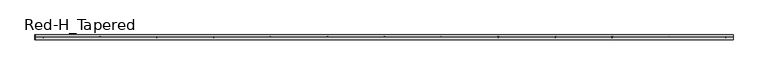
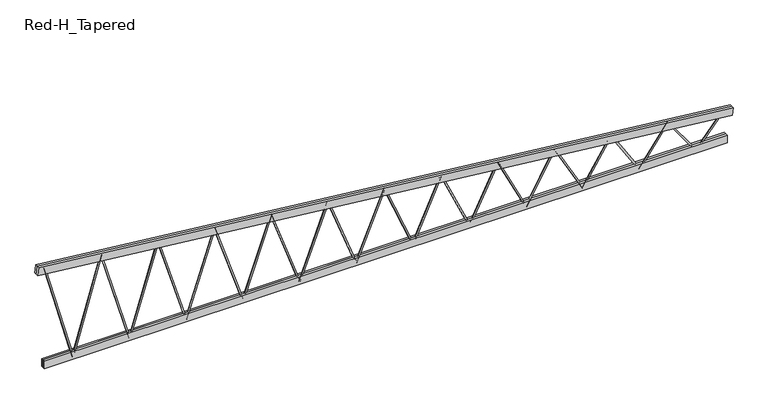
"""IFC4 building model written with IfcOpenShell, lengths in millimetres: beam geometry, Construction_Frames_RedBuilt_Openweb_Red-H_Tapered : Red-H_Tapered."""

from ifc_helpers import new_model, si_unit, point, frame, origin, origin_2d, place, context, project, spatial, polyline, circle_curve, trimmed, segment, composite_curve, outline, extrude, source, transform, mapped, element, save


def red_h_tapered_b2b48a9a(model_context):
    return source(origin(), model_context, "Body", "SweptSolid", [
        extrude(outline(composite_curve([segment(trimmed(circle_curve(origin_2d(), 12.7), [point((0.0, -12.7))], [point((0.0, 12.7))], False, "CARTESIAN"), True, "CONTINUOUS"), segment(trimmed(circle_curve(origin_2d(), 12.7), [point((0.0, 12.7))], [point((0.0, -12.7))], False, "CARTESIAN"), True, "CONTINUOUS")], self_intersect=False)), frame((-491.6619792, 0.0, -367.0101562), z_axis=(-0.35578994847905354, 0.0, 0.9345659487490824), x_axis=(0.0, -1.0, 0.0)), (0.0, 0.0, 1.0), 1381.888334),
        extrude(outline(composite_curve([segment(trimmed(circle_curve(origin_2d(), 12.7), [point((0.0, 12.7))], [point((0.0, -12.6999999))], False, "CARTESIAN"), True, "CONTINUOUS"), segment(trimmed(circle_curve(origin_2d(), 12.7), [point((0.0, -12.6999999))], [point((0.0, 12.7))], False, "CARTESIAN"), True, "CONTINUOUS")], self_intersect=False)), frame((-1474.9859375, 0.0, -367.0101562), z_axis=(0.3557899484790537, 0.0, 0.9345659487490823), x_axis=(0.0, -1.0, 0.0)), (0.0, 0.0, 1.0), 1381.888334),
        extrude(outline(composite_curve([segment(trimmed(circle_curve(origin_2d(), 12.7), [point((0.0, -12.7))], [point((0.0, 12.6999999))], False, "CARTESIAN"), True, "CONTINUOUS"), segment(trimmed(circle_curve(origin_2d(), 12.7), [point((0.0, 12.6999999))], [point((0.0, -12.7))], False, "CARTESIAN"), True, "CONTINUOUS")], self_intersect=False)), frame((-1474.9859375, 0.0, -367.0101562), z_axis=(-0.3329345647396236, 0.0, 0.9429499327120382), x_axis=(0.0, -1.0, 0.0)), (0.0, 0.0, 1.0), 1476.7525852),
        extrude(outline(composite_curve([segment(trimmed(circle_curve(origin_2d(), 12.7), [point((0.0, -12.7))], [point((0.0, 12.7))], False, "CARTESIAN"), True, "CONTINUOUS"), segment(trimmed(circle_curve(origin_2d(), 12.7), [point((0.0, 12.7))], [point((0.0, -12.7))], False, "CARTESIAN"), True, "CONTINUOUS")], self_intersect=False)), frame((-2458.3098958, 0.0, -367.0101562), z_axis=(0.3329345647396277, 0.0, 0.9429499327120368), x_axis=(0.0, -1.0, 0.0)), (0.0, 0.0, 1.0), 1476.7525852),
        extrude(outline(composite_curve([segment(trimmed(circle_curve(origin_2d(), 12.7), [point((0.0, 12.7))], [point((0.0, -12.7))], False, "CARTESIAN"), True, "CONTINUOUS"), segment(trimmed(circle_curve(origin_2d(), 12.7), [point((0.0, -12.7))], [point((0.0, 12.7))], False, "CARTESIAN"), True, "CONTINUOUS")], self_intersect=False)), frame((-2458.3098958, 0.0, -367.0101562), z_axis=(-0.31268525401434294, 0.0, 0.9498567954812904), x_axis=(0.0, -1.0, 0.0)), (0.0, 0.0, 1.0), 1572.3862026),
        extrude(outline(composite_curve([segment(trimmed(circle_curve(origin_2d(), 12.7), [point((0.0, -12.7))], [point((0.0, 12.7))], False, "CARTESIAN"), True, "CONTINUOUS"), segment(trimmed(circle_curve(origin_2d(), 12.7), [point((0.0, 12.7))], [point((0.0, -12.7))], False, "CARTESIAN"), True, "CONTINUOUS")], self_intersect=False)), frame((-3441.6338542, 0.0, -367.0101562), z_axis=(0.31268525401434244, 0.0, 0.9498567954812905), x_axis=(0.0, -1.0, 0.0)), (0.0, 0.0, 1.0), 1572.3862026),
        extrude(outline(composite_curve([segment(trimmed(circle_curve(origin_2d(), 12.7), [point((0.0, 12.7))], [point((0.0, -12.7))], False, "CARTESIAN"), True, "CONTINUOUS"), segment(trimmed(circle_curve(origin_2d(), 12.7), [point((0.0, -12.7))], [point((0.0, 12.7))], False, "CARTESIAN"), True, "CONTINUOUS")], self_intersect=False)), frame((-3441.6338542, 0.0, -367.0101562), z_axis=(-0.2946453378709869, 0.0, 0.9556066789589177), x_axis=(0.0, -1.0, 0.0)), (0.0, 0.0, 1.0), 1668.6569104),
        extrude(outline(composite_curve([segment(trimmed(circle_curve(origin_2d(), 12.7), [point((0.0, -12.7))], [point((0.0, 12.7))], False, "CARTESIAN"), True, "CONTINUOUS"), segment(trimmed(circle_curve(origin_2d(), 12.7), [point((0.0, 12.7))], [point((0.0, -12.7))], False, "CARTESIAN"), True, "CONTINUOUS")], self_intersect=False)), frame((-4424.9578125, 0.0, -367.0101562), z_axis=(0.29464533787099256, 0.0, 0.9556066789589159), x_axis=(0.0, -1.0, 0.0)), (0.0, 0.0, 1.0), 1668.6569104),
        extrude(outline(composite_curve([segment(trimmed(circle_curve(origin_2d(), 12.7), [point((0.0, 12.7))], [point((0.0, -12.7))], False, "CARTESIAN"), True, "CONTINUOUS"), segment(trimmed(circle_curve(origin_2d(), 12.7), [point((0.0, -12.7))], [point((0.0, 12.7))], False, "CARTESIAN"), True, "CONTINUOUS")], self_intersect=False)), frame((-4424.9578125, 0.0, -367.0101562), z_axis=(-0.2784893697457482, 0.0, 0.9604393114292105), x_axis=(0.0, -1.0, 0.0)), (0.0, 0.0, 1.0), 1765.46049),
        extrude(outline(composite_curve([segment(trimmed(circle_curve(origin_2d(), 12.7), [point((0.0, -12.7))], [point((0.0, 12.6999999))], False, "CARTESIAN"), True, "CONTINUOUS"), segment(trimmed(circle_curve(origin_2d(), 12.7), [point((0.0, 12.6999999))], [point((0.0, -12.7))], False, "CARTESIAN"), True, "CONTINUOUS")], self_intersect=False)), frame((-5408.2817708, 0.0, -367.0101562), z_axis=(0.27848936974574684, 0.0, 0.9604393114292109), x_axis=(0.0, -1.0, 0.0)), (0.0, 0.0, 1.0), 1765.46049),
        extrude(outline(composite_curve([segment(trimmed(circle_curve(origin_2d(), 12.7), [point((0.0, 12.7))], [point((0.0, -12.7000001))], False, "CARTESIAN"), True, "CONTINUOUS"), segment(trimmed(circle_curve(origin_2d(), 12.7), [point((0.0, -12.7000001))], [point((0.0, 12.7))], False, "CARTESIAN"), True, "CONTINUOUS")], self_intersect=False)), frame((-5408.2817708, 0.0, -367.0101562), z_axis=(-0.2639492777400827, 0.0, 0.9645365616608262), x_axis=(0.0, -1.0, 0.0)), (0.0, 0.0, 1.0), 1862.7138645),
        extrude(outline(composite_curve([segment(trimmed(circle_curve(origin_2d(), 12.7), [point((0.0, 12.7000001))], [point((0.0, -12.6999999))], False, "CARTESIAN"), True, "CONTINUOUS"), segment(trimmed(circle_curve(origin_2d(), 12.7), [point((0.0, -12.6999999))], [point((0.0, 12.7000001))], False, "CARTESIAN"), True, "CONTINUOUS")], self_intersect=False)), frame((5408.2817708, 0.0, -367.0101562), z_axis=(0.6439089672678159, 0.0, 0.7651021120557013), x_axis=(0.0, -1.0, 0.0)), (0.0, 0.0, 1.0), 763.5582111),
        extrude(outline(composite_curve([segment(trimmed(circle_curve(origin_2d(), 12.7), [point((0.0, -12.7))], [point((0.0, 12.7))], False, "CARTESIAN"), True, "CONTINUOUS"), segment(trimmed(circle_curve(origin_2d(), 12.7), [point((0.0, 12.7))], [point((0.0, -12.7))], False, "CARTESIAN"), True, "CONTINUOUS")], self_intersect=False)), frame((5408.2817708, 0.0, -367.0101562), z_axis=(-0.582969105772275, 0.0, 0.8124943210355837), x_axis=(0.0, -1.0, 0.0)), (0.0, 0.0, 1.0), 843.3757026),
        extrude(outline(composite_curve([segment(trimmed(circle_curve(origin_2d(), 12.7), [point((0.0, 12.7000001))], [point((0.0, -12.7))], False, "CARTESIAN"), True, "CONTINUOUS"), segment(trimmed(circle_curve(origin_2d(), 12.7), [point((0.0, -12.7))], [point((0.0, 12.7000001))], False, "CARTESIAN"), True, "CONTINUOUS")], self_intersect=False)), frame((4424.9578125, 0.0, -367.0101562), z_axis=(0.5829691057722728, 0.0, 0.8124943210355852), x_axis=(0.0, -1.0, 0.0)), (0.0, 0.0, 1.0), 843.3757026),
        extrude(outline(composite_curve([segment(trimmed(circle_curve(origin_2d(), 12.7), [point((0.0, -12.7))], [point((0.0, 12.6999999))], False, "CARTESIAN"), True, "CONTINUOUS"), segment(trimmed(circle_curve(origin_2d(), 12.7), [point((0.0, 12.6999999))], [point((0.0, -12.7))], False, "CARTESIAN"), True, "CONTINUOUS")], self_intersect=False)), frame((4424.9578125, 0.0, -367.0101562), z_axis=(-0.530184660192729, 0.0, 0.8478822006011923), x_axis=(0.0, -1.0, 0.0)), (0.0, 0.0, 1.0), 927.3410117),
        extrude(outline(composite_curve([segment(trimmed(circle_curve(origin_2d(), 12.7), [point((0.0, 12.7))], [point((0.0, -12.7))], False, "CARTESIAN"), True, "CONTINUOUS"), segment(trimmed(circle_curve(origin_2d(), 12.7), [point((0.0, -12.7))], [point((0.0, 12.7))], False, "CARTESIAN"), True, "CONTINUOUS")], self_intersect=False)), frame((3441.6338542, 0.0, -367.0101562), z_axis=(0.5301846601927269, 0.0, 0.8478822006011937), x_axis=(0.0, -1.0, 0.0)), (0.0, 0.0, 1.0), 927.3410117),
        extrude(outline(composite_curve([segment(trimmed(circle_curve(origin_2d(), 12.7), [point((0.0, -12.7))], [point((0.0, 12.7))], False, "CARTESIAN"), True, "CONTINUOUS"), segment(trimmed(circle_curve(origin_2d(), 12.7), [point((0.0, 12.7))], [point((0.0, -12.7))], False, "CARTESIAN"), True, "CONTINUOUS")], self_intersect=False)), frame((3441.6338542, 0.0, -367.0101562), z_axis=(-0.48467074935534127, 0.0, 0.8746966701201806), x_axis=(0.0, -1.0, 0.0)), (0.0, 0.0, 1.0), 1014.4246993),
        extrude(outline(composite_curve([segment(trimmed(circle_curve(origin_2d(), 12.7), [point((0.0, 12.7))], [point((0.0, -12.7))], False, "CARTESIAN"), True, "CONTINUOUS"), segment(trimmed(circle_curve(origin_2d(), 12.7), [point((0.0, -12.7))], [point((0.0, 12.7))], False, "CARTESIAN"), True, "CONTINUOUS")], self_intersect=False)), frame((2458.3098958, 0.0, -367.0101562), z_axis=(0.48467074935534193, 0.0, 0.8746966701201804), x_axis=(0.0, -1.0, 0.0)), (0.0, 0.0, 1.0), 1014.4246993),
        extrude(outline(composite_curve([segment(trimmed(circle_curve(origin_2d(), 12.7), [point((0.0, -12.7))], [point((0.0, 12.7))], False, "CARTESIAN"), True, "CONTINUOUS"), segment(trimmed(circle_curve(origin_2d(), 12.7), [point((0.0, 12.7))], [point((0.0, -12.7))], False, "CARTESIAN"), True, "CONTINUOUS")], self_intersect=False)), frame((2458.3098958, 0.0, -367.0101562), z_axis=(-0.4453907754718369, 0.0, 0.8953362815861959), x_axis=(0.0, -1.0, 0.0)), (0.0, 0.0, 1.0), 1103.8890032),
        extrude(outline(composite_curve([segment(trimmed(circle_curve(origin_2d(), 12.7), [point((0.0, 12.7))], [point((0.0, -12.7))], False, "CARTESIAN"), True, "CONTINUOUS"), segment(trimmed(circle_curve(origin_2d(), 12.7), [point((0.0, -12.7))], [point((0.0, 12.7))], False, "CARTESIAN"), True, "CONTINUOUS")], self_intersect=False)), frame((1474.9859375, 0.0, -367.0101562), z_axis=(0.445390775471841, 0.0, 0.8953362815861938), x_axis=(0.0, -1.0, 0.0)), (0.0, 0.0, 1.0), 1103.8890032),
        extrude(outline(composite_curve([segment(trimmed(circle_curve(origin_2d(), 12.7), [point((0.0, -12.7))], [point((0.0, 12.7))], False, "CARTESIAN"), True, "CONTINUOUS"), segment(trimmed(circle_curve(origin_2d(), 12.7), [point((0.0, 12.7))], [point((0.0, -12.7))], False, "CARTESIAN"), True, "CONTINUOUS")], self_intersect=False)), frame((1474.9859375, 0.0, -367.0101562), z_axis=(-0.41136395902525497, 0.0, 0.9114711697114004), x_axis=(0.0, -1.0, 0.0)), (0.0, 0.0, 1.0), 1195.1994539),
        extrude(outline(composite_curve([segment(trimmed(circle_curve(origin_2d(), 12.7), [point((0.0, 12.7))], [point((0.0, -12.7))], False, "CARTESIAN"), True, "CONTINUOUS"), segment(trimmed(circle_curve(origin_2d(), 12.7), [point((0.0, -12.7))], [point((0.0, 12.7))], False, "CARTESIAN"), True, "CONTINUOUS")], self_intersect=False)), frame((491.6619792, 0.0, -367.0101562), z_axis=(0.41136395902525574, 0.0, 0.9114711697114), x_axis=(0.0, -1.0, 0.0)), (0.0, 0.0, 1.0), 1195.1994539),
        extrude(outline(composite_curve([segment(trimmed(circle_curve(origin_2d(), 12.7), [point((0.0, -12.7))], [point((0.0, 12.7))], False, "CARTESIAN"), True, "CONTINUOUS"), segment(trimmed(circle_curve(origin_2d(), 12.7), [point((0.0, 12.7))], [point((0.0, -12.7))], False, "CARTESIAN"), True, "CONTINUOUS")], self_intersect=False)), frame((491.6619792, 0.0, -367.0101562), z_axis=(-0.3817359681353622, 0.0, 0.9242714161066314), x_axis=(0.0, -1.0, 0.0)), (0.0, 0.0, 1.0), 1287.9634622),
        extrude(outline(composite_curve([segment(trimmed(circle_curve(origin_2d(), 12.7), [point((0.0, 12.7))], [point((0.0, -12.7))], False, "CARTESIAN"), True, "CONTINUOUS"), segment(trimmed(circle_curve(origin_2d(), 12.7), [point((0.0, -12.7))], [point((0.0, 12.7))], False, "CARTESIAN"), True, "CONTINUOUS")], self_intersect=False)), frame((-491.6619792, 0.0, -367.0101562), z_axis=(0.3817359681353307, 0.0, 0.9242714161066444), x_axis=(0.0, -1.0, 0.0)), (0.0, 0.0, 1.0), 1287.9634622),
        extrude(outline(polyline([(-5925.34375, -41.275), (-5925.34375, -3.175), (5925.34375, -3.175), (5925.34375, -41.275), (-5925.34375, -41.275)])), frame((0.0, 0.0, -386.0601562), z_axis=(0.0, 0.0, 1.0), x_axis=(1.0, 0.0, 0.0)), (0.0, 0.0, 1.0), 139.7),
        extrude(outline(polyline([(-5925.34375, 3.175), (-5925.34375, 41.275), (5925.34375, 41.275), (5925.34375, 3.175), (-5925.34375, 3.175)])), frame((0.0, 0.0, -386.0601562), z_axis=(0.0, 0.0, 1.0), x_axis=(1.0, 0.0, 0.0)), (0.0, 0.0, 1.0), 139.7),
        extrude(outline(polyline([(0.0, -38.1), (0.0, 0.0), (12121.9438686, 0.0), (12121.9438686, -38.1), (0.0, -38.1)])), frame((-6041.7262958, -3.175, 1367.3241631), z_axis=(0.10581636195546858, 0.0, 0.9943856885245832), x_axis=(0.9943856885245832, 0.0, -0.10581636195546858)), (0.0, 0.0, 1.0), 139.7),
        extrude(outline(polyline([(0.0, -38.1), (0.0, 0.0), (12121.9438686, 0.0), (12121.9438686, -38.1), (0.0, -38.1)])), frame((-6041.7262958, 41.275, 1367.3241631), z_axis=(0.10581636195546858, 0.0, 0.9943856885245832), x_axis=(0.9943856885245832, 0.0, -0.10581636195546858)), (0.0, 0.0, 1.0), 139.7),
    ])


if __name__ == "__main__":
    model = new_model("IFC4")
    model_context = context("Model", 3, world=origin())
    ifc_project = project(units=[si_unit("LENGTHUNIT", "METRE", prefix="MILLI")], contexts=[model_context])
    site = spatial("IfcSite", under=ifc_project)
    building = spatial("IfcBuilding", under=site)
    placement = place(None, origin())
    red_h_tapered_shape = red_h_tapered_b2b48a9a(model_context)
    element("IfcBeam", 1, ObjectType="Construction_Frames_RedBuilt_Openweb_Red-H_Tapered : Red-H_Tapered", at=placement, inside=building, context=model_context, shape_type="MappedRepresentation", body=[
        mapped(red_h_tapered_shape, transform((0.0, 0.0, 0.0), x_axis=(1.0, 0.0, 0.0), y_axis=(0.0, 1.0, 0.0), z_axis=(0.0, 0.0, 1.0))),
    ])
    save(model, "model.ifc")

# Revit data of these elements
# Type "Construction_Frames_RedBuilt_Openweb_Red-H_Tapered : Red-H_Tapered"
#   Youtube clip = ""
#   Weight Net (Kg) = "0"
#   Webs = "Up to 2\" diameter tubular steel"
#   Uniformat II Description = ""
#   Uniformat II Code = ""
#   Uniclass 2015 Name = "Softwood trusses"
#   Uniclass 2015 Code = "Pr_20_85_90_81"
#   Uniclass 2.0 Description = "Structural Framing Systems"
#   Uniclass 2.0 Code = "SS-15-10-75"
#   Uniclass 1.4 Description = "Trusses"
#   Uniclass 1.4 Code = "L3523"
#   UNSPSC Code = "30103606"
#   Technical description = "http://www.redbuilt.com/reference/literature-and-other-resources"
#   Region South America = "None"
#   Region Oceania = "None"
#   Region North America = "US"
#   Region Middle East = "None"
#   Region Europe = "None"
#   Region Asia = "None"
#   Region Antarctica = "None"
#   Region Africa = "None"
#   QR code = "http://bimobject.com/redbuilt/product/redbuilt-0003"
#   Product url = "http://www.redbuilt.com/products/default.aspx?id=2"
#   Product group = "Wood Trusses"
#   Product family = "Construction"
#   Product data url = "https://bimobject.com/redbuilt/product/redbuilt-0003"
#   Product certification = ""
#   Product SKU = "redbuilt-0003"
#   Product Page URL = "http://www.redbuilt.com/commercial-systems/red-m-red-h-open-web-trusses"
#   Product Guid = "2c5793f2-6ffb-4665-b825-cf90c048e711"
#   Product Documentation Link = "http://www.redbuilt.com/documents/OW_Guide_2017_07_LowRes_wLinks.pdf"
#   OmniClass Description = "Wood Trusses"
#   OmniClass Code = "23-13 35 19 13 17"
#   NBS Reference Description = ""
#   NBS Reference Code = ""
#   Material secondary = "Steel"
#   Material main = "Wood"
#   Masterformat 2014 Description = "Metal-Web Wood Joists"
#   Masterformat 2014 Code = "06 17 36"
#   Manufacturer name = "RedBuilt"
#   Manufacturer country = "United States"
#   Installation instructions = "http://www.redbuilt.com/documents/Installation_Sheets_Open-Web.pdf"
#   IFC Classification = ""
#   EAN code = ""
#   Design country = "United States"
#   Product Information = "http://redbuilt.com/products/default.aspx?id=2"
#   Model = "Red-H-Tapered"
#   Manufacturer URL = "http://redbuilt.com/"
#   Manufacturer = "RedBuilt™"
#   Description = "Open Web Truss"
#   Date of publishing = "8/17/2010"
#   Contact us = "http://redbuilt.com/contact/"
#   Chords = "Double 1½\" x 5½\" MSR lumber"
#   COBIe Type Category = ""
#   Brand url = "http://www.redbuilt.com"
#   BIMobject main category code = "construction"
#   BIMobject main category = "Construction"
#   BIMobject category code = "construction-frames-trusses"
#   BIMobject category = "Frames & Trusses"
#   Web Radius = 0' - 0 1/2"
#   Web Layout Offset Start [instance default] = 0' - 5"
#   Web Layout Offset End [instance default] = 0' - 5"
#   Web Diameter = 0' - 1"
#   TotalLength [instance default] = 20' - 0"
#   Span Minimum = 4' - 0"
#   Span Maximum = 70' - 0"
#   Span Limit [instance default] = 20' - 0"
#   Nominal width = 0' - 0"
#   Nominal height = 0' - 0"
#   Inner Depth Top [instance default] = 0' - 2.76372"
#   Depth Start [instance default] = 6' - 0"
#   Top Chord Length [instance default] = 20' - 1.19701"
#   TC Extension Start Aux [instance default] = 0' - 0"
#   TC Extension End Aux [instance default] = 0' - 0"
#   T-B Chord Length Difference L [instance default] = 0' - 4"
#   T-B Chord Length Difference [instance default] = 0' - 4"
#   Height 2 [instance default] = 6' - 0"
#   Depth Minimum at Wall = 2' - 0"
#   Depth Maximum at Wall = 6' - 0"
#   Depth Lower End [instance default] = 2' - 0"
#   Depth Higher End [instance default] = 6' - 0"
#   Depth End [instance default] = 2' - 0"
#   Depth 2 [instance default] = 2' - 0"
#   Chord Width = 0' - 3 1/4"
#   Chord Thickness = 0' - 1 1/2"
#   Chord Depth = 0' - 5 1/2"
#   Offset Start [instance default] = 0' - 0"
#   TC Extension Start [instance default] = 0' - 0"
#   End Panel = 0' - 5"
#   Offset End [instance default] = 0' - 0"
#   TC Extension End [instance default] = 0' - 0"
#   Length [instance default] = 20' - 0"
#   Angle [instance default] = 5.71059°
#   Span Limit Warning [instance default] = no
#   Edition number = 1
#   Top Bearing Start [instance default] = yes
#   Top Bearing End [instance default] = yes
#   Bottom Bearing Start [instance default] = no
#   Bottom Bearing End [instance default] = no
#   8 Panels [instance default] = yes
#   16 Panels [instance default] = no
#   12 Panels [instance default] = no
#   Web Material = RedBuilt-Steel, Galvanized
#   Clip Material = RedBuilt-Steel, Galvanized
#   Chords Material = RedBuilt-MSR
#   URL = ""
#   Assembly Code = ""
# Element 1 (IfcBeam, "Construction_Frames_RedBuilt_Openweb_Red-H_Tapered : Red-H_Tapered")
#   TotalLength = 39' - 6 9/16"
#   Span Limit = 39' - 6 9/16"
#   Inner Depth Top = 0' - 2.76553"
#   Depth Start = 4' - 0"
#   Top Chord Length = 39' - 9.24188"
#   Height 2 = 4' - 0"
#   Depth Higher End = 4' - 0"
#   Depth 2 = 4' - 2 1/2"
#   Angle = 6.0742°
#   8 Panels = no
#   12 Panels = yes
#   Materials on its faces: "RedBuilt-Steel, Galvanized", "RedBuilt-MSR"
# Materials
#   "RedBuilt-Steel, Galvanized": class "Metal", colour RGB 164 172 176, transparency 0, Manufacturer = "RedBuilt. LLC", Comments = "Openweb Metal Web", URL = "http://www.redbuilt.com/", Description = "Galvanized steel", Cost = 0
#   "RedBuilt-MSR": class "Wood", colour RGB 213 182 136, transparency 0, Manufacturer = "RedBuilt, LLC", URL = "http://www.redbuilt.com/", Cost = 0
